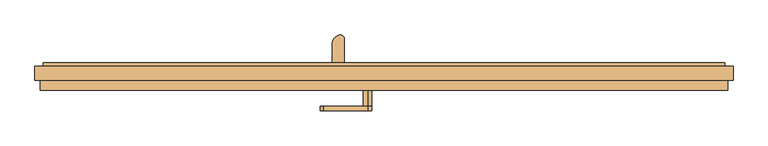
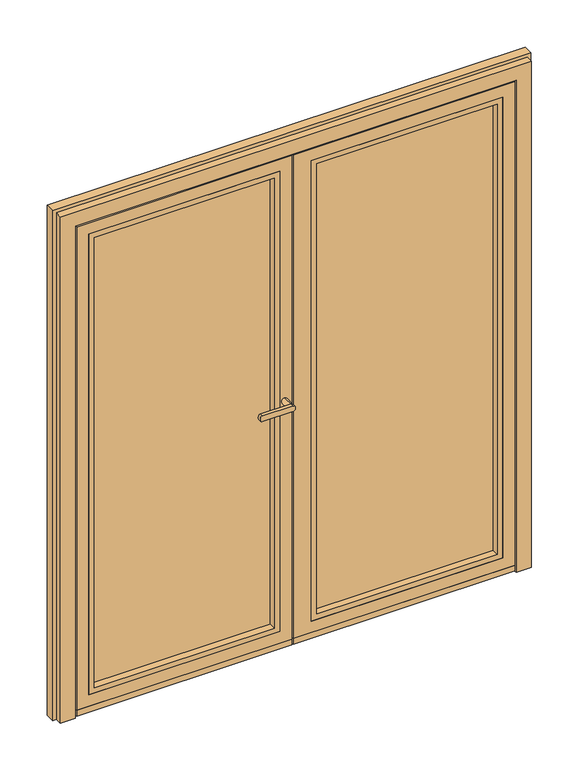
"""IFC4 building model written with IfcOpenShell, lengths in millimetres: door geometry, Schueco_FWS_ADS-75-HD-HI_out_Family-02 : FWS SI insert unit."""

from ifc_helpers import new_model, si_unit, point, frame, frame_2d, origin, place, context, project, spatial, polyline, circle_curve, ellipse_curve, trimmed, segment, composite_curve, outline, extrude, faceted_brep, source, transform, mapped, element, save
from ifc_brep_helpers import plane_surface, cylinder_surface, extruded_surface, advanced_brep


def door_162ddc2b(model_context):
    return source(origin(), model_context, "Body", "SolidModel", [
        faceted_brep([(875.0, -57.4997281, 33.0), (875.0, -57.4997281, 2075.0), (875.0, -66.0000038, 2075.0), (875.0, -66.0000038, 33.0), (-10.0, -66.0000038, 33.0), (-10.0, -57.4997281, 33.0), (5.0, -57.4997281, 33.0), (885.0, -57.4997281, 23.0), (885.0, -57.4997281, 2085.0), (5.0, -57.4997281, 2085.0), (5.0, -57.4997281, 2075.0), (5.0, -57.4997281, 23.0), (-10.0, -66.0000038, 2075.0), (63.0, -66.0000038, 81.0), (63.0, -66.0000038, 2027.0), (827.0, -66.0000038, 2027.0), (827.0, -66.0000038, 81.0), (827.0, 0.5000388, 2027.0), (827.0, 0.5000388, 81.0), (63.0, 0.5000388, 81.0), (63.0, 0.5000388, 2027.0), (88.0, 0.5000388, 106.0), (88.0, 0.5000388, 2002.0), (802.0, 0.5000388, 2002.0), (802.0, 0.5000388, 106.0), (802.0, 8.9999962, 2002.0), (802.0, 8.9999962, 106.0), (88.0, 8.9999962, 106.0), (88.0, 8.9999962, 2002.0), (900.0, 8.9999962, 8.0), (15.0, 8.9999962, 8.0), (15.0, 8.9999962, 2100.0), (900.0, 8.9999962, 2100.0), (900.0, 0.5000388, 2100.0), (900.0, 0.5000388, 8.0), (15.0, 0.5000388, 8.0), (15.0, 0.5000388, 2100.0), (15.0, 0.5000388, 2085.0), (885.0, 0.5000388, 2085.0), (885.0, 0.5000388, 23.0), (15.0, 0.5000388, 23.0), (5.0, 0.5000388, 23.0), (5.0, 0.5000388, 2085.0), (-10.0, -57.4997281, 2075.0)], [[[0, 1, 2, 3]], [[3, 4, 5, 6, 0]], [[7, 8, 9, 10, 1, 0, 6, 11]], [[2, 12, 4, 3], [13, 14, 15, 16]], [[16, 15, 17, 18]], [[18, 19, 13, 16]], [[19, 20, 14, 13]], [[18, 17, 20, 19], [21, 22, 23, 24]], [[24, 23, 25, 26]], [[26, 27, 21, 24]], [[27, 28, 22, 21]], [[29, 30, 31, 32], [26, 25, 28, 27]], [[29, 32, 33, 34]], [[34, 35, 30, 29]], [[33, 36, 37, 38, 39, 40, 35, 34]], [[39, 38, 8, 7]], [[7, 11, 41, 40, 39]], [[11, 6, 10, 9, 42, 41]], [[1, 10, 43, 12, 2]], [[20, 17, 15, 14]], [[28, 25, 23, 22]], [[32, 31, 36, 33]], [[9, 8, 38, 37, 42]], [[43, 10, 6, 5]], [[4, 12, 43, 5]], [[37, 36, 31, 30, 35, 40]], [[40, 41, 42, 37]]]),
        extrude(outline(polyline([(81.0, 63.0), (81.0, 827.0), (2027.0, 827.0), (2027.0, 63.0), (81.0, 63.0)]), holes=[polyline([(103.0, 805.0), (103.0, 85.0), (2005.0, 85.0), (2005.0, 805.0), (103.0, 805.0)])]), frame((0.0, -66.0000038, 0.0), z_axis=(0.0, 1.0, 0.0), x_axis=(0.0, 0.0, 1.0)), (0.0, 0.0, 1.0), 28.5000426),
        extrude(outline(polyline([(63.0, -37.4999612), (63.0, 0.5000388), (827.0, 0.5000388), (827.0, -37.4999612), (63.0, -37.4999612)])), frame((0.0, 0.0, 81.0), z_axis=(0.0, 0.0, 1.0), x_axis=(1.0, 0.0, 0.0)), (0.0, 0.0, 1.0), 1946.0),
        extrude(outline(composite_curve([segment(polyline([(-52.7483946, 4.2956275), (-52.7483946, 23.0), (-31.443662, 23.0), (-31.443662, 4.2956275)]), True, "CONTINUOUS"), segment(trimmed(circle_curve(frame_2d((-42.0960283, 15.355415)), 15.3555139), [point((-31.443662, 4.2956275))], [point((-52.7483946, 4.2956275))], False, "CARTESIAN"), True, "CONTINUOUS")], self_intersect=False)), frame((5.0, 0.0, 0.0), z_axis=(1.0, 0.0, 0.0), x_axis=(0.0, 1.0, 0.0)), (0.0, 0.0, 1.0), 880.0),
        extrude(outline(polyline([(875.0, -66.0000038), (-10.0, -66.0000038), (-10.0, -57.4997281), (875.0, -57.4997281), (875.0, -66.0000038)])), frame((0.0, 0.0, 8.0), z_axis=(0.0, 0.0, 1.0), x_axis=(1.0, 0.0, 0.0)), (0.0, 0.0, 1.0), 25.0),
        extrude(outline(composite_curve([segment(polyline([(-141.6673236, 8.9997177), (-141.6673236, 59.1618682)]), True, "CONTINUOUS"), segment(trimmed(circle_curve(frame_2d((-114.4889059, 59.1618682)), 27.1784177), [point((-141.6673236, 59.1618682))], [point((-124.0260015, 84.6120194))], False, "CARTESIAN"), True, "CONTINUOUS"), segment(trimmed(circle_curve(frame_2d((-119.9485005, 73.7310321)), 11.6198924), [point((-124.0260015, 84.6120194))], [point((-108.3286081, 73.7310321))], False, "CARTESIAN"), True, "CONTINUOUS"), segment(polyline([(-108.3286081, 73.7310321), (-108.3286081, 8.9997177), (-141.6673236, 8.9997177)]), True, "CONTINUOUS")], self_intersect=False)), frame((0.0, 0.0, 2043.9340013), z_axis=(0.0, 0.0, 1.0), x_axis=(1.0, 0.0, 0.0)), (0.0, 0.0, 1.0), 4.0),
        extrude(outline(polyline([(-141.6673236, 12.9997177), (-108.3286081, 12.9997177), (-108.3286081, 8.9997177), (-141.6673236, 8.9997177), (-141.6673236, 12.9997177)])), frame((0.0, 0.0, 2013.9340013), z_axis=(0.0, 0.0, 1.0), x_axis=(1.0, 0.0, 0.0)), (0.0, 0.0, 1.0), 30.0),
        extrude(outline(polyline([(-141.6673236, 12.9997177), (-108.3286081, 12.9997177), (-108.3286081, 8.9997177), (-141.6673236, 8.9997177), (-141.6673236, 12.9997177)])), frame((0.0, 0.0, 56.9340013), z_axis=(0.0, 0.0, 1.0), x_axis=(1.0, 0.0, 0.0)), (0.0, 0.0, 1.0), 30.0),
        extrude(outline(composite_curve([segment(polyline([(-141.6673236, 8.9997177), (-141.6673236, 59.1618682)]), True, "CONTINUOUS"), segment(trimmed(circle_curve(frame_2d((-114.4889059, 59.1618682)), 27.1784177), [point((-141.6673236, 59.1618682))], [point((-124.0260015, 84.6120194))], False, "CARTESIAN"), True, "CONTINUOUS"), segment(trimmed(circle_curve(frame_2d((-119.9485005, 73.7310321)), 11.6198924), [point((-124.0260015, 84.6120194))], [point((-108.3286081, 73.7310321))], False, "CARTESIAN"), True, "CONTINUOUS"), segment(polyline([(-108.3286081, 73.7310321), (-108.3286081, 8.9997177), (-141.6673236, 8.9997177)]), True, "CONTINUOUS")], self_intersect=False)), frame((0.0, 0.0, 52.9340013), z_axis=(0.0, 0.0, 1.0), x_axis=(1.0, 0.0, 0.0)), (0.0, 0.0, 1.0), 4.0),
        advanced_brep(
        [(-112.282924, 57.5977179, 2043.9340013), (-137.717076, 72.2821425, 2043.9340013), (-112.282924, 57.5977179, 56.9340013), (-137.717076, 72.2821425, 56.9340013)],
        [
            (0, 1, ellipse_curve(frame((-125.0, 64.9399302, 2043.9340013), z_axis=(0.0, 0.0, 1.0000000000000002), x_axis=(0.5000002582658958, 0.866025254674503, 0.0)), 21.5840887, 14.6844171)),
            (1, 0, ellipse_curve(frame((-125.0, 64.9399302, 2043.9340013), z_axis=(0.0, 0.0, 1.0000000000000002), x_axis=(0.5000002582658958, 0.866025254674503, 0.0)), 21.5840887, 14.6844171)),
            (2, 3, ellipse_curve(frame((-125.0, 64.9399302, 56.9340013), z_axis=(0.0, 0.0, -1.0000000000000002), x_axis=(-0.866025254674503, 0.5000002582658958, 0.0)), 14.6844171, 21.5840887)),
            (3, 2, ellipse_curve(frame((-125.0, 64.9399302, 56.9340013), z_axis=(0.0, 0.0, -1.0000000000000002), x_axis=(-0.866025254674503, 0.5000002582658958, 0.0)), 14.6844171, 21.5840887)),
            (0, 2),
            (3, 1),
        ],
        [
            plane_surface(frame((-137.717076, 72.2821425, 2043.9340013), z_axis=(0.0, 0.0, 1.0000000000000002), x_axis=(0.5000002582658958, 0.866025254674503, 0.0))),
            plane_surface(frame((-137.717076, 72.2821425, 56.9340013), z_axis=(0.0, 0.0, -1.0000000000000002), x_axis=(-0.5000002582658958, -0.866025254674503, 0.0))),
            extruded_surface(trimmed(ellipse_curve(frame((-125.0, 64.9399302, 56.9340013), z_axis=(0.0, 0.0, -1.0000000000000002), x_axis=(-0.866025254674503, 0.5000002582658958, 0.0)), 14.6844171, 21.5840887), [point((-137.717076, 72.2821425, 56.9340013))], [point((-112.282924, 57.5977179, 56.9340013))], True, "CARTESIAN"), (0.0, 0.0, -1987.0), 1987.0),
            extruded_surface(trimmed(ellipse_curve(frame((-125.0, 64.9399302, 56.9340013), z_axis=(0.0, 0.0, -1.0000000000000002), x_axis=(-0.866025254674503, 0.5000002582658958, 0.0)), 14.6844171, 21.5840887), [point((-112.282924, 57.5977179, 56.9340013))], [point((-137.717076, 72.2821425, 56.9340013))], True, "CARTESIAN"), (0.0, 0.0, -1987.0), 1987.0),
        ],
        [
            (0, [[1, 2]]),
            (1, [[3, 4]]),
            (2, [[5, -4, 6, -1]]),
            (3, [[-6, -3, -5, -2]]),
        ],
    ),
        advanced_brep(
        [(-45.0, -122.0002518, 1038.0113692), (-45.0, -122.0002518, 1061.9886308), (-166.6617926, -122.0002518, 1061.9886308), (-166.6617926, -122.0002518, 1038.0113692), (-45.0, -109.5001648, 1061.9886308), (-45.0, -109.5001648, 1038.0113692), (-166.6617926, -109.5001648, 1038.0113692), (-166.6617926, -109.5001648, 1061.9886308), (-45.0, -66.0002823, 1038.0113692), (-45.0, -66.0002823, 1061.9886308)],
        [
            (0, 1, circle_curve(frame((-45.0, -122.0002518, 1050.0), z_axis=(0.0, -1.0, 0.0), x_axis=(0.0, 0.0, 1.0)), 11.9886308)),
            (1, 2),
            (2, 3, ellipse_curve(frame((-166.6617926, -122.0002518, 1050.0), z_axis=(0.0, -1.0, 0.0), x_axis=(0.0, 0.0, -1.0)), 11.9886308, 7.9050795)),
            (3, 0),
            (4, 5, circle_curve(frame((-45.0, -109.5001648, 1050.0), z_axis=(0.0, -1.0, 0.0), x_axis=(0.0, 0.0, 1.0)), 11.9886308)),
            (5, 6),
            (6, 7, ellipse_curve(frame((-166.6617926, -109.5001648, 1050.0), z_axis=(0.0, 1.0, 0.0), x_axis=(0.0, 0.0, -1.0)), 11.9886308, 7.9050795)),
            (7, 4),
            (3, 6),
            (5, 0),
            (2, 7),
            (1, 4),
            (5, 4, circle_curve(frame((-45.0, -109.5001648, 1050.0), z_axis=(0.0, -1.0, 0.0), x_axis=(0.0, 0.0, 1.0)), 11.9886308)),
            (8, 9, circle_curve(frame((-45.0, -66.0002823, 1050.0), z_axis=(0.0, 1.0, 0.0), x_axis=(0.0, 0.0, 1.0)), 11.9886308)),
            (9, 8, circle_curve(frame((-45.0, -66.0002823, 1050.0), z_axis=(0.0, 1.0, 0.0), x_axis=(0.0, 0.0, 1.0)), 11.9886308)),
            (8, 5),
            (4, 9),
        ],
        [
            plane_surface(frame((-166.6617926, -122.0002518, 1038.0113692), z_axis=(0.0, -1.0, 0.0), x_axis=(-1.0, 0.0, 0.0))),
            plane_surface(frame((-166.6617926, -109.5001648, 1038.0113692), z_axis=(0.0, 1.0, 0.0), x_axis=(1.0, 0.0, 0.0))),
            plane_surface(frame((-45.0, -122.0002518, 1038.0113692), z_axis=(0.0, 0.0, -1.0), x_axis=(0.0, 1.0, 0.0))),
            extruded_surface(trimmed(ellipse_curve(frame((-166.6617926, -109.5001648, 1050.0), z_axis=(0.0, 1.0, 0.0), x_axis=(0.0, 0.0, -1.0)), 11.9886308, 7.9050795), [point((-166.6617926, -109.5001648, 1038.0113692))], [point((-166.6617926, -109.5001648, 1061.9886308))], True, "CARTESIAN"), (0.0, 12.500086999999994, 0.0), 12.500086999999994),
            plane_surface(frame((-166.6617926, -122.0002518, 1061.9886308), z_axis=(0.0, 0.0, 1.0), x_axis=(0.0, 1.0, 0.0))),
            cylinder_surface(frame((-45.0, -109.5001648, 1050.0), z_axis=(0.0, -1.0, 0.0), x_axis=(0.0, 0.0, 1.0)), 11.9886308),
            plane_surface(frame((-45.0, -66.0002823, 1061.9886308), z_axis=(0.0, 1.0, 0.0), x_axis=(-1.0, 0.0, 0.0))),
            cylinder_surface(frame((-45.0, -66.0002823, 1050.0), z_axis=(0.0, -1.0, 0.0), x_axis=(0.0, 0.0, 1.0)), 11.9886308),
        ],
        [
            (0, [[1, 2, 3, 4]]),
            (1, [[5, 6, 7, 8]]),
            (2, [[9, -6, 10, -4]]),
            (3, [[11, -7, -9, -3]]),
            (4, [[12, -8, -11, -2]]),
            (5, [[-10, 13, -12, -1]]),
            (6, [[14, 15]]),
            (7, [[16, -5, 17, -14]]),
            (7, [[-17, -13, -16, -15]]),
        ],
    ),
        faceted_brep([(-875.0, -57.5000065, 33.0), (-875.0, -66.0002823, 33.0), (-875.0, -66.0002823, 2075.0), (-875.0, -57.5000065, 2075.0), (-17.0, -57.5000065, 33.0), (-15.0, -57.5000065, 33.0), (-15.0, -66.0002823, 33.0), (-17.0, -66.0002823, 33.0), (-885.0, -57.5000065, 23.0), (-5.0, -57.5000065, 23.0), (-5.0, -57.5000065, 2085.0), (-885.0, -57.5000065, 2085.0), (-15.0, -57.5000065, 2075.0), (-17.0, -57.5000065, 2075.0), (-15.0, -66.0002823, 2075.0), (-17.0, -66.0002823, 2075.0), (-63.0, -66.0002823, 81.0), (-827.0, -66.0002823, 81.0), (-827.0, -66.0002823, 2027.0), (-63.0, -66.0002823, 2027.0), (-827.0, 0.4997603, 81.0), (-827.0, 0.4997603, 2027.0), (-63.0, 0.4997603, 81.0), (-63.0, 0.4997603, 2027.0), (-88.0, 0.4997603, 106.0), (-802.0, 0.4997603, 106.0), (-802.0, 0.4997603, 2002.0), (-88.0, 0.4997603, 2002.0), (-802.0, 8.9997177, 106.0), (-802.0, 8.9997177, 2002.0), (-88.0, 8.9997177, 106.0), (-88.0, 8.9997177, 2002.0), (10.0, 8.9997177, 8.0), (-900.0, 8.9997177, 8.0), (-900.0, 8.9997177, 2100.0), (10.0, 8.9997177, 2100.0), (-900.0, 0.4997603, 8.0), (-900.0, 0.4997603, 2100.0), (10.0, 0.4997603, 8.0), (10.0, 0.4997603, 2100.0), (-5.0, 0.4997603, 23.0), (-885.0, 0.4997603, 23.0), (-885.0, 0.4997603, 2085.0), (-5.0, 0.4997603, 2085.0)], [[[0, 1, 2, 3]], [[1, 0, 4, 5, 6, 7]], [[8, 9, 10, 11], [12, 5, 4, 0, 3, 13]], [[6, 5, 12, 14]], [[6, 14, 15, 2, 1, 7], [16, 17, 18, 19]], [[17, 20, 21, 18]], [[20, 17, 16, 22]], [[22, 16, 19, 23]], [[20, 22, 23, 21], [24, 25, 26, 27]], [[25, 28, 29, 26]], [[28, 25, 24, 30]], [[30, 24, 27, 31]], [[32, 33, 34, 35], [28, 30, 31, 29]], [[33, 36, 37, 34]], [[36, 33, 32, 38]], [[38, 32, 35, 39]], [[36, 38, 39, 37], [40, 41, 42, 43]], [[41, 8, 11, 42]], [[8, 41, 40, 9]], [[9, 40, 43, 10]], [[14, 12, 13, 3, 2, 15]], [[23, 19, 18, 21]], [[31, 27, 26, 29]], [[39, 35, 34, 37]], [[10, 43, 42, 11]]]),
        extrude(outline(polyline([(81.0, -63.0), (2027.0, -63.0), (2027.0, -827.0), (81.0, -827.0), (81.0, -63.0)]), holes=[polyline([(103.0, -805.0), (2005.0, -805.0), (2005.0, -85.0), (103.0, -85.0), (103.0, -805.0)])]), frame((0.0, -66.0002823, 0.0), z_axis=(0.0, 1.0, 0.0), x_axis=(0.0, 0.0, 1.0)), (0.0, 0.0, 1.0), 28.5000426),
        extrude(outline(polyline([(-63.0, -37.5002397), (-827.0, -37.5002397), (-827.0, 0.4997603), (-63.0, 0.4997603), (-63.0, -37.5002397)])), frame((0.0, 0.0, 81.0), z_axis=(0.0, 0.0, 1.0), x_axis=(1.0, 0.0, 0.0)), (0.0, 0.0, 1.0), 1946.0),
        extrude(outline(composite_curve([segment(polyline([(-52.748673, 4.2956275), (-52.748673, 23.0), (-31.4439405, 23.0), (-31.4439405, 4.2956275)]), True, "CONTINUOUS"), segment(trimmed(circle_curve(frame_2d((-42.0963068, 15.355415)), 15.3555139), [point((-31.4439405, 4.2956275))], [point((-52.748673, 4.2956275))], False, "CARTESIAN"), True, "CONTINUOUS")], self_intersect=False)), frame((-885.0, 0.0, 0.0), z_axis=(1.0, 0.0, 0.0), x_axis=(0.0, 1.0, 0.0)), (0.0, 0.0, 1.0), 880.0),
        extrude(outline(polyline([(-875.0, -66.0002823), (-875.0, -57.5000065), (-15.0, -57.5000065), (-15.0, -66.0002823), (-875.0, -66.0002823)])), frame((0.0, 0.0, 8.0), z_axis=(0.0, 0.0, 1.0), x_axis=(1.0, 0.0, 0.0)), (0.0, 0.0, 1.0), 25.0),
        faceted_brep([(930.999943, 8.9997177, 2130.999943), (930.999943, 0.0, 2130.999943), (930.999943, 0.0, 0.0), (930.999943, 8.9997177, 0.0), (-954.0, 0.0, 0.0), (-954.0, 0.0, 2154.0), (954.0, 0.0, 2154.0), (954.0, 0.0, 0.0), (-930.999943, 0.0, 2130.999943), (-930.999943, 0.0, 0.0), (954.0, -38.0, 0.0), (940.0, -38.0, 0.0), (940.0, -66.0002823, 0.0), (880.0652914, -66.0002823, 0.0), (880.0652914, -57.5000065, 0.0), (893.4999114, -57.5000065, 0.0), (893.4999114, 0.4997603, 0.0), (904.9999827, 0.4997603, 0.0), (904.9999827, 8.9997177, 0.0), (-904.9999827, 8.9997177, 0.0), (-930.999943, 8.9997177, 0.0), (-930.999943, 8.9997177, 2130.999943), (904.9999827, 8.9997177, 2104.9999827), (-904.9999827, 8.9997177, 2104.9999827), (880.0652914, -66.0002823, 2080.0652914), (880.0652914, -57.5000065, 2080.0652914), (-880.0652914, -57.5000065, 0.0), (-893.4999114, -57.5000065, 0.0), (-893.4999114, -57.5000065, 2093.4999114), (893.4999114, -57.5000065, 2093.4999114), (-880.0652914, -57.5000065, 2080.0652914), (-940.0, -66.0002823, 0.0), (-880.0652914, -66.0002823, 0.0), (-880.0652914, -66.0002823, 2080.0652914), (940.0, -66.0002823, 2140.0), (-940.0, -66.0002823, 2140.0), (940.0, -38.0, 2140.0), (-954.0, -38.0, 0.0), (-940.0, -38.0, 0.0), (-940.0, -38.0, 2140.0), (954.0, -38.0, 2154.0), (-954.0, -38.0, 2154.0), (-904.9999827, 0.4997603, 0.0), (-893.4999114, 0.4997603, 0.0), (904.9999827, 0.4997603, 2104.9999827), (-904.9999827, 0.4997603, 2104.9999827), (893.4999114, 0.4997603, 2093.4999114), (-893.4999114, 0.4997603, 2093.4999114)], [[[0, 1, 2, 3]], [[4, 5, 6, 7, 2, 1, 8, 9]], [[3, 2, 7, 10, 11, 12, 13, 14, 15, 16, 17, 18]], [[19, 20, 21, 0, 3, 18, 22, 23]], [[24, 25, 14, 13]], [[26, 27, 28, 29, 15, 14, 25, 30]], [[31, 32, 33, 24, 13, 12, 34, 35]], [[34, 12, 11, 36]], [[37, 38, 39, 36, 11, 10, 40, 41]], [[4, 9, 20, 19, 42, 43, 27, 26, 32, 31, 38, 37]], [[20, 9, 8, 21]], [[18, 17, 44, 22]], [[42, 19, 23, 45]], [[32, 26, 30, 33]], [[31, 35, 39, 38]], [[4, 37, 41, 5]], [[6, 40, 10, 7]], [[43, 42, 45, 44, 17, 16, 46, 47]], [[16, 15, 29, 46]], [[27, 43, 47, 28]], [[21, 8, 1, 0]], [[33, 30, 25, 24]], [[35, 34, 36, 39]], [[23, 22, 44, 45]], [[5, 41, 40, 6]], [[47, 46, 29, 28]]]),
    ])


if __name__ == "__main__":
    model = new_model("IFC4")
    model_context = context("Model", 3, world=origin())
    ifc_project = project(units=[si_unit("LENGTHUNIT", "METRE", prefix="MILLI")], contexts=[model_context])
    site = spatial("IfcSite", under=ifc_project)
    building = spatial("IfcBuilding", under=site)
    placement = place(None, origin())
    door_shape = door_162ddc2b(model_context)
    element("IfcDoor", 1, ObjectType="Schueco_FWS_ADS-75-HD-HI_out_Family-02 : FWS SI insert unit", at=placement, inside=building, context=model_context, shape_type="MappedRepresentation", body=[
        mapped(door_shape, transform((0.0, 0.0, 0.0), x_axis=(1.0, 0.0, 0.0), y_axis=(0.0, 1.0, 0.0), z_axis=(0.0, 0.0, 1.0))),
    ])
    save(model, "model.ifc")

# Revit data of these elements
# Type "Schueco_FWS_ADS-75-HD-HI_out_Family-02 : FWS SI insert unit"
#   Type Mark = "52"
#   __NOTE__ = "Data describes the optimum values of the entire system. The properites of a selected design option have to be determined on an individual basis!"
#   Wind load resistance = "Class 2"
#   Watertightness = "Class 5A"
#   Thermal insulation = "Uf = 1.4 W/(m²K)"
#   Sound insulation = "Rw 43 dB"
#   Schueco thermal insulation standard = "Highly thermally insulated"
#   Opening type = "Outward-opening, Flush-fitted"
#   Model = "Schueco ADS 75 HD.HI"
#   Mechanical loading = "Class 2"
#   Maximum leaf width in mm = "1400"
#   Maximum leaf weight in kg = "200"
#   Maximum leaf height in mm = "3000"
#   Material = "Aluminium"
#   Long term functionality = "Class 6"
#   Construction Type = "Door, double-leaf, outward-opening"
#   Manufacturer = "Schueco International KG"
#   Glazing data = "Triple glazing 38mm"
#   Façade insert unit = "yes"
#   Family creation date = "08.2017"
#   Description = "Schueco Aluminium Door System (ADS)"
#   Burglar resistance = "Class RC 3"
#   Areas of use = "Public buildings"
#   Analytic Construction = "<None>"
#   Air permeability = "Class 2"
#   Width [instance default] = 997.866 mm
#   Leaf opening angle [instance default] = 0.00°
#   IOf_T = 38 mm
#   Height [instance default] = 2054.517 mm
#   Glazing area [instance default] = 0.930355 m²
#   F2_W [instance default] = 498.933 mm
#   F1_W [instance default] = 498.933 mm
#   Distance from bottom to handles [instance default] = 1050 mm
#   Clear opening width [instance default] = 849.866 mm
#   Active leaf width = 1100 mm
#   Standard threshold = no
#   Low level threshold = yes
#   Handles = yes
#   FWS SI insert unit = yes
#   FWS HI insert unit = no
#   All fields of identical width = yes
#   Glass = none
#   Frame = Alu
#   Fittings = none
# Element 1 (IfcDoor, "Schueco_FWS_ADS-75-HD-HI_out_Family-02 : FWS SI insert unit")
#   Width = 1908 mm
#   Height = 2154 mm
#   Glazing area = 2.70749 m²
#   F2_W = 954 mm
#   F1_W = 954 mm
#   Clear opening width = 1760 mm
#   Materials on its faces: "Alu", "Glass"
# Materials
#   "Alu": class "Glas", colour RGB 140 140 140, transparency 0
#   "Glass": class "Glass", colour RGB 128 128 255, transparency 0.75, Description = "Soda Lime Glass", Cost = 0
